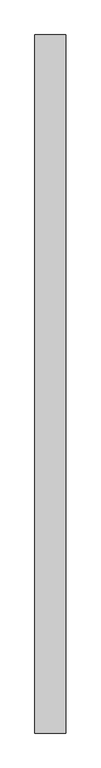
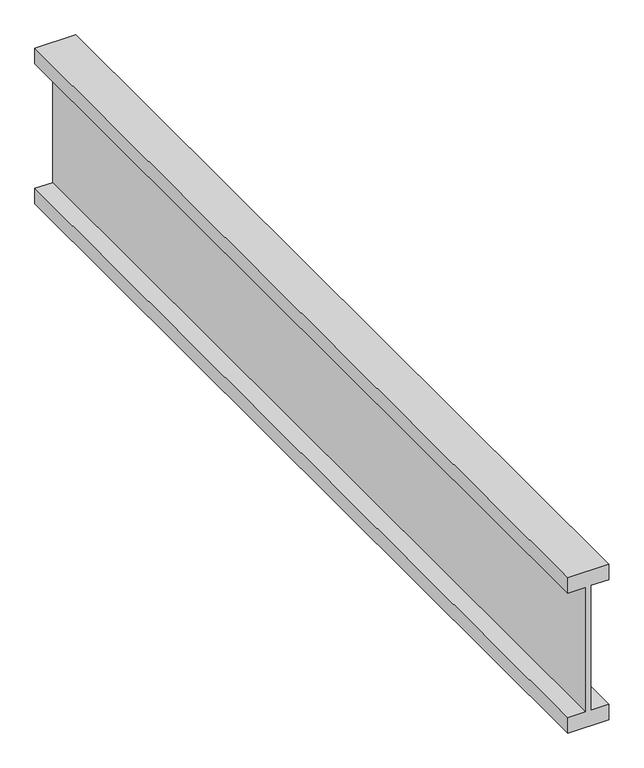
"""IFC4 building model written with IfcOpenShell, lengths in millimetres: proxy geometry, Framing065 7730 : Framing065 7730."""

import ifcopenshell
import ifcopenshell.guid

model = None  # the IFC model being written
_history = None  # IfcOwnerHistory: only IFC2X3 demands one
_inside = {}  # id of a spatial element -> (the spatial element, [elements in it])
_under = {}  # id of a project, library or spatial element -> (it, [spatial elements below it])
_declared = {}  # id of a project -> (the project, [libraries it declares])
_typed = {}  # id of a type object -> (the type object, [elements of that type])
_made_of = {}  # id of a material, layer set ... -> (it, [elements and type objects made of it])


def new_model(schema):
    """Start an empty IFC model of exactly this schema.

    Asked for "IFC4X3", IfcOpenShell would pick the latest addendum, in which some entities
    have other attributes; the version numbers below select the first issue.
    IFC2X3 requires an IfcOwnerHistory on every rooted entity: one is made here for all.
    """
    global model, _history
    if schema == "IFC4X3":
        model = ifcopenshell.file(schema_version=(4, 3, 0, 0))
    else:
        model = ifcopenshell.file(schema=schema)
    _inside.clear()
    _under.clear()
    _declared.clear()
    _typed.clear()
    _made_of.clear()
    _history = None
    if model.schema == "IFC2X3":
        org = make("IfcOrganization", Name="unknown")
        user = make(
            "IfcPersonAndOrganization",
            ThePerson=make("IfcPerson", FamilyName="unknown"),
            TheOrganization=org,
        )
        app = make(
            "IfcApplication",
            ApplicationDeveloper=org,
            Version="unknown",
            ApplicationFullName="unknown",
            ApplicationIdentifier="unknown",
        )
        _history = make(
            "IfcOwnerHistory",
            OwningUser=user,
            OwningApplication=app,
            ChangeAction="ADDED",
            CreationDate=0,
        )
    return model


def make(cls, **values):
    """One entity of the class cls with the attributes given. An attribute that is None is left unset."""
    return model.create_entity(
        cls, **{name: value for name, value in values.items() if value is not None}
    )


def rooted(cls, **values):
    """An entity with a GlobalId (a new one), such as an element, a storey or a relation."""
    return make(cls, GlobalId=ifcopenshell.guid.new(), OwnerHistory=_history, **values)


def si_unit(unit_type, name, prefix=None):
    """IfcSIUnit, for example si_unit("LENGTHUNIT", "METRE", prefix="MILLI")."""
    return make("IfcSIUnit", UnitType=unit_type, Prefix=prefix, Name=name)


def assignment(units):
    """IfcUnitAssignment: the units of a project."""
    return None if units is None else make("IfcUnitAssignment", Units=units)


def point(xyz):
    """IfcCartesianPoint."""
    return None if xyz is None else make("IfcCartesianPoint", Coordinates=xyz)


def direction(xyz):
    """IfcDirection."""
    return None if xyz is None else make("IfcDirection", DirectionRatios=xyz)


def frame(location, z_axis=None, x_axis=None):
    """IfcAxis2Placement3D, a coordinate frame: its origin and axes. An axis left out is left unset."""
    return make(
        "IfcAxis2Placement3D",
        Location=point(location),
        Axis=direction(z_axis),
        RefDirection=direction(x_axis),
    )


def origin():
    """The frame at (0, 0, 0) with its axes left unset."""
    return frame((0.0, 0.0, 0.0))


def place(relative_to, where):
    """IfcLocalPlacement: puts the frame where relative to a parent placement (None: the world)."""
    return make(
        "IfcLocalPlacement", PlacementRelTo=relative_to, RelativePlacement=where
    )


def context(
    kind, dimensions, precision=None, world=None, true_north=None, identifier=None
):
    """IfcGeometricRepresentationContext, for example the 3D "Model" context."""
    return make(
        "IfcGeometricRepresentationContext",
        ContextIdentifier=identifier,
        ContextType=kind,
        CoordinateSpaceDimension=dimensions,
        Precision=precision,
        WorldCoordinateSystem=world,
        TrueNorth=true_north,
    )


def project(units=None, contexts=None):
    """IfcProject with its units and contexts."""
    return rooted(
        "IfcProject",
        Name="project",
        RepresentationContexts=contexts,
        UnitsInContext=assignment(units),
    )


def spatial(cls, under=None, at=None, **own):
    """A site, building, storey or space (cls), placed at a placement, below another one or the project."""
    s = rooted(cls, ObjectPlacement=at, **own)
    if under is not None:
        _under.setdefault(under.id(), (under, []))[1].append(s)
    return s


def polyline(points):
    """IfcPolyline through the points."""
    return make("IfcPolyline", Points=[point(p) for p in points])


def outline(outer, holes=None, kind="AREA"):
    """IfcArbitraryClosedProfileDef: a profile drawn as a closed curve; with holes, ...WithVoids."""
    if holes is None:
        return make("IfcArbitraryClosedProfileDef", ProfileType=kind, OuterCurve=outer)
    return make(
        "IfcArbitraryProfileDefWithVoids",
        ProfileType=kind,
        OuterCurve=outer,
        InnerCurves=holes,
    )


def extrude(swept, where, along, depth):
    """IfcExtrudedAreaSolid: the profile swept, set in the frame where, extruded along a direction by depth."""
    return make(
        "IfcExtrudedAreaSolid",
        SweptArea=swept,
        Position=where,
        ExtrudedDirection=direction(along),
        Depth=depth,
    )


def shape(context_of_items, identifier, shape_type, items):
    """IfcShapeRepresentation: the items that make up one representation, for example the "Body"."""
    return make(
        "IfcShapeRepresentation",
        ContextOfItems=context_of_items,
        RepresentationIdentifier=identifier,
        RepresentationType=shape_type,
        Items=items,
    )


def source(mapping_origin, context_of_items, identifier, shape_type, items):
    """IfcRepresentationMap: a shape defined once, which mapped items show again and again."""
    return make(
        "IfcRepresentationMap",
        MappingOrigin=mapping_origin,
        MappedRepresentation=shape(context_of_items, identifier, shape_type, items),
    )


def transform(
    local_origin,
    x_axis=None,
    y_axis=None,
    z_axis=None,
    scale=None,
    scale2=None,
    scale3=None,
    uniform=True,
):
    """IfcCartesianTransformationOperator3D, or its non-uniform kind. x_axis, y_axis, z_axis: its Axis1, 2, 3."""
    if uniform:
        return make(
            "IfcCartesianTransformationOperator3D",
            Axis1=direction(x_axis),
            Axis2=direction(y_axis),
            LocalOrigin=point(local_origin),
            Scale=scale,
            Axis3=direction(z_axis),
        )
    return make(
        "IfcCartesianTransformationOperator3DnonUniform",
        Axis1=direction(x_axis),
        Axis2=direction(y_axis),
        LocalOrigin=point(local_origin),
        Scale=scale,
        Axis3=direction(z_axis),
        Scale2=scale2,
        Scale3=scale3,
    )


def mapped(mapping_source, mapping_target):
    """IfcMappedItem: shows the shape of a source again, moved by a transform."""
    return make(
        "IfcMappedItem", MappingSource=mapping_source, MappingTarget=mapping_target
    )


def made_of(thing, what):
    """Note that an element or type object is made of a material, layer set ...; save() writes the relation."""
    if what is not None:
        _made_of.setdefault(what.id(), (what, []))[1].append(thing)
    return thing


def element(
    cls,
    number,
    at=None,
    inside=None,
    cuts=None,
    type_object=None,
    material=None,
    context=None,
    identifier="Body",
    shape_type=None,
    held_by="IfcProductDefinitionShape",
    body=None,
    shapes=None,
    **own,
):
    """One element of the class cls, such as IfcWall. Its Tag is "e" and its number.

    at: its placement. inside: the storey or other place that contains it. cuts: it is an
    opening in that element (IfcRelVoidsElement). A single representation is given by context,
    identifier, shape_type and body (its items); several are given by shapes. held_by: the class
    of the entity that holds the representations. save() writes the other relations.
    """
    e = rooted(cls, Tag="e%d" % number, ObjectPlacement=at, **own)
    if body is not None:
        shapes = [shape(context, identifier, shape_type, body)]
    if shapes is not None:
        e.Representation = make(held_by, Representations=shapes)
    if inside is not None:
        _inside.setdefault(inside.id(), (inside, []))[1].append(e)
    if cuts is not None:
        rooted(
            "IfcRelVoidsElement", RelatingBuildingElement=cuts, RelatedOpeningElement=e
        )
    if type_object is not None:
        _typed.setdefault(type_object.id(), (type_object, []))[1].append(e)
    return made_of(e, material)


def aggregate(whole, parts):
    """IfcRelAggregates: a whole, such as a stair, and the parts it consists of."""
    return rooted("IfcRelAggregates", RelatingObject=whole, RelatedObjects=parts)


def save(model, path):
    """Write the relations noted so far, then the file.

    IfcRelAggregates (storeys below a building ...), IfcRelContainedInSpatialStructure (elements
    in a storey), IfcRelDefinesByType, IfcRelAssociatesMaterial and IfcRelDeclares: one each for
    every whole, place, type object, material and project.
    """
    for whole, parts in _under.values():
        aggregate(whole, parts)
    for where, things in _inside.values():
        rooted(
            "IfcRelContainedInSpatialStructure",
            RelatedElements=things,
            RelatingStructure=where,
        )
    for kind, things in _typed.values():
        rooted("IfcRelDefinesByType", RelatedObjects=things, RelatingType=kind)
    for what, things in _made_of.values():
        rooted("IfcRelAssociatesMaterial", RelatedObjects=things, RelatingMaterial=what)
    for by, libraries in _declared.values():
        rooted("IfcRelDeclares", RelatingContext=by, RelatedDefinitions=libraries)
    model.write(path)


def generic_models_252a1c86(model_context):
    return source(origin(), model_context, "Body", "SweptSolid", [
        extrude(outline(polyline([(40077.771, 8096.295938), (39792.021, 8096.295938), (39792.021, 8057.402188), (39757.096, 8057.402188), (39757.096, 8146.302188), (39792.021, 8146.302188), (39792.021, 8107.408438), (40077.771, 8107.408438), (40077.771, 8146.302188), (40112.696, 8146.302188), (40112.696, 8057.402188), (40077.771, 8057.402188), (40077.771, 8096.295938)])), frame((0.0, -3747.9491938, 0.0), z_axis=(0.0, 1.0, 0.0), x_axis=(0.0, 0.0, 1.0)), (0.0, 0.0, 1.0), 2000.0),
    ])


if __name__ == "__main__":
    model = new_model("IFC4")
    model_context = context("Model", 3, world=origin())
    ifc_project = project(units=[si_unit("LENGTHUNIT", "METRE", prefix="MILLI")], contexts=[model_context])
    site = spatial("IfcSite", under=ifc_project)
    building = spatial("IfcBuilding", under=site)
    placement = place(None, origin())
    generic_models_shape = generic_models_252a1c86(model_context)
    element("IfcBuildingElementProxy", 1, Name="Framing065 7730 : Framing065 7730", ObjectType="Framing065 7730 : Framing065 7730", at=placement, inside=building, context=model_context, shape_type="MappedRepresentation", body=[
        mapped(generic_models_shape, transform((0.0, 0.0, 0.0), x_axis=(1.0, 0.0, 0.0), y_axis=(0.0, 1.0, 0.0), z_axis=(0.0, 0.0, 1.0))),
    ])
    save(model, "model.ifc")

# Revit data of these elements
# Type "Framing065 7730 : Framing065 7730"
#   NameOverride = "Framing065"
# Element 1 (IfcBuildingElementProxy, "Framing065 7730 : Framing065 7730")
#   Materials on its faces: "WOOD FRAMING (SEE STRUCT DWGS)"
# Materials
#   "WOOD FRAMING (SEE STRUCT DWGS)": class "Unassigned", colour RGB 224 188 168, transparency 0, Cost = 0
